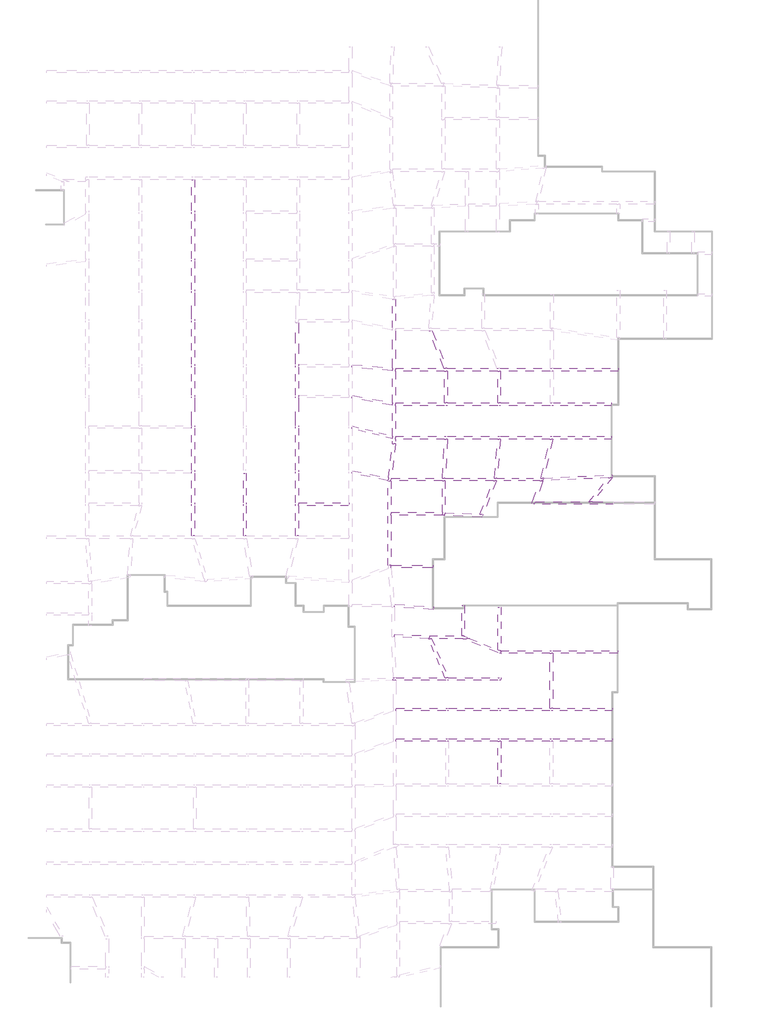
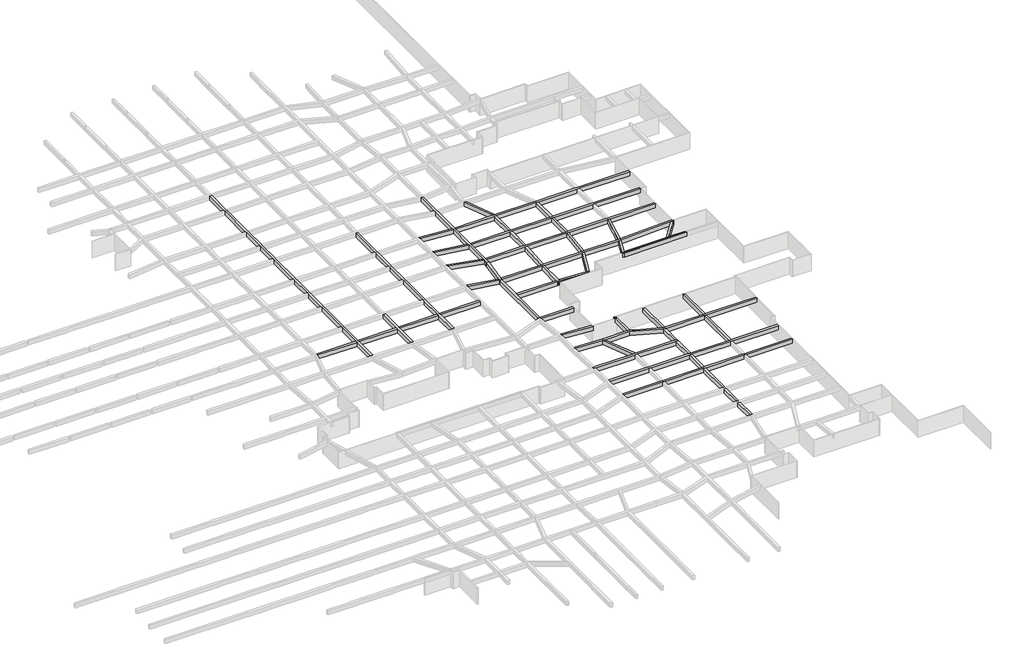
# One storey, part 24 of 45: 43 beams.
"""IFC4 building model written with IfcOpenShell, lengths in millimetres."""

from ifc_helpers import new_model, si_unit, frame, origin, place, context, project, spatial, polyline, outline, extrude, faceted_brep, element, save

model = new_model("IFC4")

# Units and contexts
model_context = context("Model", 3, world=origin())
ifc_project = project(units=[si_unit("LENGTHUNIT", "METRE", prefix="MILLI")], contexts=[model_context])

# Site, building, storey
site = spatial("IfcSite", under=ifc_project)
building = spatial("IfcBuilding", under=site)
storey = spatial("IfcBuildingStorey", under=building, Name="户型图", Elevation=0.0)

# Beams
placement = place(None, origin())
element("IfcBeam", 1, ObjectType="混凝土 - 矩形梁 : KL_beam", at=placement, inside=storey, context=model_context, shape_type="Brep", body=[
    faceted_brep([(1471.7652295, 23868.127427, 3300.0), (1071.7652295, 23868.127427, 3300.0), (1071.7652295, 19231.9876735, 3300.0), (1071.7652295, 18831.9876735, 3300.0), (1071.7652295, 12131.9876735, 3300.0), (1071.7652295, 11731.9876735, 3300.0), (1071.7652295, 7519.5822838, 3300.0), (1071.7652295, 7119.5822838, 3300.0), (1071.7652295, 3119.5822838, 3300.0), (1071.7652295, 2719.5822838, 3300.0), (1071.7652295, -3551.5199121, 3300.0), (1071.7652295, -3951.5199121, 3300.0), (1071.7652295, -8106.533538, 3300.0), (1071.7652295, -8506.533538, 3300.0), (1071.7652295, -12606.533538, 3300.0), (1071.7652295, -13006.533538, 3300.0), (1071.7652295, -19266.2432363, 3300.0), (1071.7652295, -19666.2432363, 3300.0), (1071.7652295, -24066.2432363, 3300.0), (1071.7652295, -24466.2432363, 3300.0), (1071.7652295, -28962.9587641, 3300.0), (1471.7652295, -28962.9587641, 3300.0), (1471.7652295, -24466.2432363, 3300.0), (1471.7652295, -24066.2432363, 3300.0), (1471.7652295, -19666.2432363, 3300.0), (1471.7652295, -19266.2432363, 3300.0), (1471.7652295, -13006.533538, 3300.0), (1471.7652295, -12606.533538, 3300.0), (1471.7652295, -8506.533538, 3300.0), (1471.7652295, -8106.533538, 3300.0), (1471.7652295, -3951.5199121, 3300.0), (1471.7652295, -3551.5199121, 3300.0), (1471.7652295, 2719.5822838, 3300.0), (1471.7652295, 3119.5822838, 3300.0), (1471.7652295, 7119.5822838, 3300.0), (1471.7652295, 7519.5822838, 3300.0), (1471.7652295, 11731.9876735, 3300.0), (1471.7652295, 12131.9876735, 3300.0), (1471.7652295, 18831.9876735, 3300.0), (1471.7652295, 19231.9876735, 3300.0), (1071.7652295, 23868.127427, 2500.0), (1071.7652295, 19231.9876735, 2500.0), (1071.7652295, 18831.9876735, 2500.0), (1071.7652295, 12131.9876735, 2500.0), (1071.7652295, 11731.9876735, 2500.0), (1071.7652295, 7519.5822838, 2500.0), (1071.7652295, 7119.5822838, 2500.0), (1071.7652295, 3119.5822838, 2500.0), (1071.7652295, 2719.5822838, 2500.0), (1071.7652295, -3551.5199121, 2500.0), (1071.7652295, -3951.5199121, 2500.0), (1071.7652295, -8106.533538, 2500.0), (1071.7652295, -8506.533538, 2500.0), (1071.7652295, -12606.533538, 2500.0), (1071.7652295, -13006.533538, 2500.0), (1071.7652295, -19266.2432363, 2500.0), (1071.7652295, -19666.2432363, 2500.0), (1071.7652295, -24066.2432363, 2500.0), (1071.7652295, -24466.2432363, 2500.0), (1071.7652295, -28962.9587641, 2500.0), (1471.7652295, 23868.127427, 2500.0), (1471.7652295, 19231.9876735, 2500.0), (1471.7652295, 18831.9876735, 2500.0), (1471.7652295, 12131.9876735, 2500.0), (1471.7652295, 11731.9876735, 2500.0), (1471.7652295, 7519.5822838, 2500.0), (1471.7652295, 7119.5822838, 2500.0), (1471.7652295, 3119.5822838, 2500.0), (1471.7652295, 2719.5822838, 2500.0), (1471.7652295, -3551.5199121, 2500.0), (1471.7652295, -3951.5199121, 2500.0), (1471.7652295, -8106.533538, 2500.0), (1471.7652295, -8506.533538, 2500.0), (1471.7652295, -12606.533538, 2500.0), (1471.7652295, -13006.533538, 2500.0), (1471.7652295, -19266.2432363, 2500.0), (1471.7652295, -19666.2432363, 2500.0), (1471.7652295, -24066.2432363, 2500.0), (1471.7652295, -24466.2432363, 2500.0), (1471.7652295, -28962.9587641, 2500.0)], [[[0, 1, 2, 3, 4, 5, 6, 7, 8, 9, 10, 11, 12, 13, 14, 15, 16, 17, 18, 19, 20, 21, 22, 23, 24, 25, 26, 27, 28, 29, 30, 31, 32, 33, 34, 35, 36, 37, 38, 39]], [[1, 40, 41, 42, 43, 44, 45, 46, 47, 48, 49, 50, 51, 52, 53, 54, 55, 56, 57, 58, 59, 20, 19, 18, 17, 16, 15, 14, 13, 12, 11, 10, 9, 8, 7, 6, 5, 4, 3, 2]], [[40, 60, 61, 62, 63, 64, 65, 66, 67, 68, 69, 70, 71, 72, 73, 74, 75, 76, 77, 78, 79, 59, 58, 57, 56, 55, 54, 53, 52, 51, 50, 49, 48, 47, 46, 45, 44, 43, 42, 41]], [[60, 0, 39, 38, 37, 36, 35, 34, 33, 32, 31, 30, 29, 28, 27, 26, 25, 24, 23, 22, 21, 79, 78, 77, 76, 75, 74, 73, 72, 71, 70, 69, 68, 67, 66, 65, 64, 63, 62, 61]], [[1, 0, 60, 40]], [[21, 20, 59, 79]]]),
])
element("IfcBeam", 2, ObjectType="混凝土 - 矩形梁 : KL_beam", at=placement, inside=storey, context=model_context, shape_type="Brep", body=[
    faceted_brep([(9169.3873949, -19666.2432363, 3300.0), (8769.3873949, -19666.2432363, 3300.0), (8769.3873949, -24066.2432363, 3300.0), (8769.3873949, -24466.2432363, 3300.0), (8769.3873949, -28962.9587641, 3300.0), (9169.3873949, -28962.9587641, 3300.0), (9169.3873949, -24466.2432363, 3300.0), (9169.3873949, -24066.2432363, 3300.0), (9169.3873949, -19666.2432363, 2500.0), (9169.3873949, -28962.9587641, 2500.0), (9169.3873949, -24466.2432363, 2500.0), (9169.3873949, -24066.2432363, 2500.0), (8769.3873949, -19666.2432363, 2500.0), (8769.3873949, -28962.9587641, 2500.0), (8769.3873949, -24466.2432363, 2500.0), (8769.3873949, -24066.2432363, 2500.0)], [[[0, 1, 2, 3, 4, 5, 6, 7]], [[8, 0, 7, 6, 5, 9, 10, 11]], [[12, 8, 11, 10, 9, 13, 14, 15]], [[1, 12, 15, 14, 13, 4, 3, 2]], [[1, 0, 8, 12]], [[5, 4, 13, 9]]]),
])
element("IfcBeam", 3, ObjectType="混凝土 - 矩形梁 : KL_beam", at=placement, inside=storey, context=model_context, shape_type="Brep", body=[
    faceted_brep([(16905.3597604, 2667.499527, 3300.0), (16505.3597604, 2674.481553, 3300.0), (16505.3597604, -3551.5199121, 3300.0), (16505.3597604, -3951.5199121, 3300.0), (16505.3597604, -8106.533538, 3300.0), (16505.3597604, -8506.533538, 3300.0), (16505.3597604, -12606.533538, 3300.0), (16505.3597604, -13006.533538, 3300.0), (16505.3597604, -19266.2432363, 3300.0), (16505.3597604, -19666.2432363, 3300.0), (16505.3597604, -24066.2432363, 3300.0), (16505.3597604, -24466.2432363, 3300.0), (16505.3597604, -28962.9587641, 3300.0), (16905.3597604, -28962.9587641, 3300.0), (16905.3597604, -24466.2432363, 3300.0), (16905.3597604, -24066.2432363, 3300.0), (16905.3597604, -19666.2432363, 3300.0), (16905.3597604, -19266.2432363, 3300.0), (16905.3597604, -13006.533538, 3300.0), (16905.3597604, -12606.533538, 3300.0), (16905.3597604, -8506.533538, 3300.0), (16905.3597604, -8106.533538, 3300.0), (16905.3597604, -3951.5199121, 3300.0), (16905.3597604, -3551.5199121, 3300.0), (16505.3597604, 2674.481553, 2500.0), (16505.3597604, -3551.5199121, 2500.0), (16505.3597604, -3951.5199121, 2500.0), (16505.3597604, -8106.533538, 2500.0), (16505.3597604, -8506.533538, 2500.0), (16505.3597604, -12606.533538, 2500.0), (16505.3597604, -13006.533538, 2500.0), (16505.3597604, -19266.2432363, 2500.0), (16505.3597604, -19666.2432363, 2500.0), (16505.3597604, -24066.2432363, 2500.0), (16505.3597604, -24466.2432363, 2500.0), (16505.3597604, -28962.9587641, 2500.0), (16905.3597604, 2667.499527, 2500.0), (16905.3597604, -3551.5199121, 2500.0), (16905.3597604, -3951.5199121, 2500.0), (16905.3597604, -8106.533538, 2500.0), (16905.3597604, -8506.533538, 2500.0), (16905.3597604, -12606.533538, 2500.0), (16905.3597604, -13006.533538, 2500.0), (16905.3597604, -19266.2432363, 2500.0), (16905.3597604, -19666.2432363, 2500.0), (16905.3597604, -24066.2432363, 2500.0), (16905.3597604, -24466.2432363, 2500.0), (16905.3597604, -28962.9587641, 2500.0)], [[[0, 1, 2, 3, 4, 5, 6, 7, 8, 9, 10, 11, 12, 13, 14, 15, 16, 17, 18, 19, 20, 21, 22, 23]], [[1, 24, 25, 26, 27, 28, 29, 30, 31, 32, 33, 34, 35, 12, 11, 10, 9, 8, 7, 6, 5, 4, 3, 2]], [[24, 36, 37, 38, 39, 40, 41, 42, 43, 44, 45, 46, 47, 35, 34, 33, 32, 31, 30, 29, 28, 27, 26, 25]], [[36, 0, 23, 22, 21, 20, 19, 18, 17, 16, 15, 14, 13, 47, 46, 45, 44, 43, 42, 41, 40, 39, 38, 37]], [[0, 36, 24, 1]], [[13, 12, 35, 47]]]),
])
element("IfcBeam", 4, ObjectType="混凝土 - 矩形梁 : KL_beam", at=placement, inside=storey, context=model_context, shape_type="SweptSolid", body=[
    extrude(outline(polyline([(-6328.2347705, -24466.2432363), (-6328.2347705, -24066.2432363), (1071.7652295, -24066.2432363), (1071.7652295, -24466.2432363), (-6328.2347705, -24466.2432363)])), frame((0.0, 0.0, 2500.0), z_axis=(0.0, 0.0, 1.0), x_axis=(1.0, 0.0, 0.0)), (0.0, 0.0, 1.0), 800.0),
    extrude(outline(polyline([(24442.7166646, -24066.2432363), (24442.7166646, -24466.2432363), (16905.3597604, -24466.2432363), (16905.3597604, -24066.2432363), (24442.7166646, -24066.2432363)])), frame((0.0, 0.0, 2500.0), z_axis=(0.0, 0.0, 1.0), x_axis=(1.0, 0.0, 0.0)), (0.0, 0.0, 1.0), 800.0),
    extrude(outline(polyline([(1471.7652295, -24466.2432363), (1471.7652295, -24066.2432363), (8769.3873949, -24066.2432363), (8769.3873949, -24466.2432363), (1471.7652295, -24466.2432363)])), frame((0.0, 0.0, 2500.0), z_axis=(0.0, 0.0, 1.0), x_axis=(1.0, 0.0, 0.0)), (0.0, 0.0, 1.0), 800.0),
    extrude(outline(polyline([(9169.3873949, -24466.2432363), (9169.3873949, -24066.2432363), (16505.3597604, -24066.2432363), (16505.3597604, -24466.2432363), (9169.3873949, -24466.2432363)])), frame((0.0, 0.0, 2500.0), z_axis=(0.0, 0.0, 1.0), x_axis=(1.0, 0.0, 0.0)), (0.0, 0.0, 1.0), 800.0),
])
element("IfcBeam", 5, ObjectType="混凝土 - 矩形梁 : KL_beam", at=placement, inside=storey, context=model_context, shape_type="Brep", body=[
    faceted_brep([(31293.5212654, -15309.9620605, 3300.0), (31293.5212654, -14614.9150331, 3300.0), (31293.5212654, -14214.9150331, 3300.0), (31293.5212654, -9661.6279316, 3300.0), (31293.5212654, -9261.6279316, 3300.0), (31293.5212654, -4524.63893, 3300.0), (31293.5212654, -4124.63893, 3300.0), (31293.5212654, 1446.1972666, 3300.0), (31293.5212654, 1846.1972666, 3300.0), (31293.5212654, 6125.9678564, 3300.0), (31056.9345953, 6101.1015953, 3300.0), (30993.5212654, 6111.1452801, 3300.0), (30893.5212654, 6126.9837241, 3300.0), (30893.5212654, 1908.2546983, 3300.0), (30893.5212654, 1500.7680203, 3300.0), (30893.5212654, -4097.664429, 3300.0), (30893.5212654, -4499.192364, 3300.0), (30893.5212654, -9205.644515, 3300.0), (30893.5212654, -9611.8151597, 3300.0), (30893.5212654, -14158.9267066, 3300.0), (30893.5212654, -14571.1721584, 3300.0), (30893.5212654, -15285.4970125, 3300.0), (30893.5212654, 6126.9837241, 2500.0), (30893.5212654, 1908.2546983, 2500.0), (30893.5212654, 1500.7680203, 2500.0), (30893.5212654, -4097.664429, 2500.0), (30893.5212654, -4499.192364, 2500.0), (30893.5212654, -9205.644515, 2500.0), (30893.5212654, -9611.8151597, 2500.0), (30893.5212654, -14158.9267066, 2500.0), (30893.5212654, -14571.1721584, 2500.0), (30893.5212654, -15285.4970125, 2500.0), (31293.5212654, 6125.9678564, 2500.0), (31293.5212654, 1846.1972666, 2500.0), (31293.5212654, 1446.1972666, 2500.0), (31293.5212654, -4124.63893, 2500.0), (31293.5212654, -4524.63893, 2500.0), (31293.5212654, -9261.6279316, 2500.0), (31293.5212654, -9661.6279316, 2500.0), (31293.5212654, -14214.9150331, 2500.0), (31293.5212654, -14614.9150331, 2500.0), (31293.5212654, -15309.9620605, 2500.0), (30993.5212654, 6111.1452801, 2500.0), (31056.9345953, 6101.1015953, 2500.0)], [[[0, 1, 2, 3, 4, 5, 6, 7, 8, 9, 10, 11, 12, 13, 14, 15, 16, 17, 18, 19, 20, 21]], [[21, 20, 19, 18, 17, 16, 15, 14, 13, 12, 22, 23, 24, 25, 26, 27, 28, 29, 30, 31]], [[32, 33, 34, 35, 36, 37, 38, 39, 40, 41, 31, 30, 29, 28, 27, 26, 25, 24, 23, 22, 42, 43]], [[9, 8, 7, 6, 5, 4, 3, 2, 1, 0, 41, 40, 39, 38, 37, 36, 35, 34, 33, 32]], [[10, 9, 32, 43]], [[22, 12, 11, 10, 43, 42]], [[0, 21, 31, 41]]]),
])
element("IfcBeam", 6, ObjectType="混凝土 - 矩形梁 : KL_beam", at=placement, inside=storey, context=model_context, shape_type="Brep", body=[
    faceted_brep([(30613.5574676, -20847.8227882, 3300.0), (30620.19498, -20793.7645877, 3300.0), (30669.3088044, -20393.7645877, 3300.0), (31293.5212654, -15309.9620605, 3300.0), (30893.5212654, -15285.4970125, 3300.0), (30270.8784709, -20356.5156317, 3300.0), (30222.0116965, -20754.503571, 3300.0), (30213.5574676, -20823.3577402, 3300.0), (30893.5212654, -15285.4970125, 2500.0), (30270.8784709, -20356.5156317, 2500.0), (30222.0116965, -20754.503571, 2500.0), (30213.5574676, -20823.3577402, 2500.0), (31293.5212654, -15309.9620605, 2500.0), (30669.3088044, -20393.7645877, 2500.0), (30620.19498, -20793.7645877, 2500.0), (30613.5574676, -20847.8227882, 2500.0)], [[[0, 1, 2, 3, 4, 5, 6, 7]], [[7, 6, 5, 4, 8, 9, 10, 11]], [[11, 10, 9, 8, 12, 13, 14, 15]], [[3, 2, 1, 0, 15, 14, 13, 12]], [[3, 12, 8, 4]], [[0, 7, 11, 15]]]),
])
element("IfcBeam", 7, ObjectType="混凝土 - 矩形梁 : KL_beam", at=placement, inside=storey, context=model_context, shape_type="Brep", body=[
    faceted_brep([(30613.5574676, -33326.8580756, 3300.0), (30613.5574676, -33322.5859731, 3300.0), (30613.5574676, -25893.7645877, 3300.0), (30613.5574676, -25493.7645877, 3300.0), (30613.5574676, -20847.8227882, 3300.0), (30213.5574676, -20823.3577402, 3300.0), (30213.5574676, -33322.5859731, 3300.0), (30213.5574676, -33344.3224528, 3300.0), (30213.5574676, -20823.3577402, 2500.0), (30213.5574676, -33322.5859731, 2500.0), (30213.5574676, -33344.3224528, 2500.0), (30613.5574676, -20847.8227882, 2500.0), (30613.5574676, -25493.7645877, 2500.0), (30613.5574676, -25893.7645877, 2500.0), (30613.5574676, -33322.5859731, 2500.0), (30613.5574676, -33326.8580756, 2500.0)], [[[0, 1, 2, 3, 4, 5, 6, 7]], [[7, 6, 5, 8, 9, 10]], [[10, 9, 8, 11, 12, 13, 14, 15]], [[4, 3, 2, 1, 0, 15, 14, 13, 12, 11]], [[4, 11, 8, 5]], [[0, 7, 10, 15]]]),
])
element("IfcBeam", 8, ObjectType="混凝土 - 矩形梁 : KL_beam", at=placement, inside=storey, context=model_context, shape_type="SweptSolid", body=[
    extrude(outline(polyline([(24842.7166646, -3969.8155562), (24842.7166646, -3568.2876212), (30893.5212654, -4097.664429), (30893.5212654, -4499.192364), (24842.7166646, -3969.8155562)])), frame((0.0, 0.0, 2500.0), z_axis=(0.0, 0.0, 1.0), x_axis=(1.0, 0.0, 0.0)), (0.0, 0.0, 1.0), 800.0),
])
element("IfcBeam", 9, ObjectType="混凝土 - 矩形梁 : KL_beam", at=placement, inside=storey, context=model_context, shape_type="Brep", body=[
    faceted_brep([(64358.9998045, -4124.63893, 3300.0), (64358.9998045, -4524.63893, 3300.0), (64358.9998045, -4524.63893, 2500.0), (64358.9998045, -4124.63893, 2500.0), (54693.5212654, -4124.63893, 3300.0), (54293.5212654, -4124.63893, 3300.0), (46792.4867011, -4124.63893, 3300.0), (46362.3003567, -4124.63893, 3300.0), (38929.4075897, -4124.63893, 3300.0), (38499.2212453, -4124.63893, 3300.0), (31293.5212654, -4124.63893, 3300.0), (31293.5212654, -4524.63893, 3300.0), (38593.5212654, -4524.63893, 3300.0), (38993.5212654, -4524.63893, 3300.0), (46493.5212654, -4524.63893, 3300.0), (46893.5212654, -4524.63893, 3300.0), (54293.5212654, -4524.63893, 3300.0), (54693.5212654, -4524.63893, 3300.0), (31293.5212654, -4524.63893, 2500.0), (38593.5212654, -4524.63893, 2500.0), (38993.5212654, -4524.63893, 2500.0), (46493.5212654, -4524.63893, 2500.0), (46893.5212654, -4524.63893, 2500.0), (54293.5212654, -4524.63893, 2500.0), (54693.5212654, -4524.63893, 2500.0), (31293.5212654, -4124.63893, 2500.0), (38499.2212453, -4124.63893, 2500.0), (38929.4075897, -4124.63893, 2500.0), (46362.3003567, -4124.63893, 2500.0), (46792.4867011, -4124.63893, 2500.0), (54293.5212654, -4124.63893, 2500.0), (54693.5212654, -4124.63893, 2500.0)], [[[0, 1, 2, 3]], [[1, 0, 4, 5, 6, 7, 8, 9, 10, 11, 12, 13, 14, 15, 16, 17]], [[2, 1, 17, 16, 15, 14, 13, 12, 11, 18, 19, 20, 21, 22, 23, 24]], [[3, 2, 24, 23, 22, 21, 20, 19, 18, 25, 26, 27, 28, 29, 30, 31]], [[0, 3, 31, 30, 29, 28, 27, 26, 25, 10, 9, 8, 7, 6, 5, 4]], [[11, 10, 25, 18]]]),
])
element("IfcBeam", 10, ObjectType="混凝土 - 矩形梁 : KL_beam", at=placement, inside=storey, context=model_context, shape_type="SweptSolid", body=[
    extrude(outline(polyline([(24842.7166646, -8544.8950536), (24842.7166646, -8138.7244089), (30893.5212654, -9205.644515), (30893.5212654, -9611.8151597), (24842.7166646, -8544.8950536)])), frame((0.0, 0.0, 2500.0), z_axis=(0.0, 0.0, 1.0), x_axis=(1.0, 0.0, 0.0)), (0.0, 0.0, 1.0), 800.0),
])
element("IfcBeam", 11, ObjectType="混凝土 - 矩形梁 : KL_beam", at=placement, inside=storey, context=model_context, shape_type="Brep", body=[
    faceted_brep([(63358.9998045, -9261.6279316, 3300.0), (63358.9998045, -9661.6279316, 3300.0), (63358.9998045, -9661.6279316, 2500.0), (63358.9998045, -9261.6279316, 2500.0), (54693.5212654, -9261.6279316, 3300.0), (54293.5212654, -9261.6279316, 3300.0), (46893.5212654, -9261.6279316, 3300.0), (46493.5212654, -9261.6279316, 3300.0), (38993.5212654, -9261.6279316, 3300.0), (38593.5212654, -9261.6279316, 3300.0), (31293.5212654, -9261.6279316, 3300.0), (31293.5212654, -9661.6279316, 3300.0), (38593.5212654, -9661.6279316, 3300.0), (38993.5212654, -9661.6279316, 3300.0), (46493.5212654, -9661.6279316, 3300.0), (46893.5212654, -9661.6279316, 3300.0), (54293.5212654, -9661.6279316, 3300.0), (54693.5212654, -9661.6279316, 3300.0), (31293.5212654, -9661.6279316, 2500.0), (38593.5212654, -9661.6279316, 2500.0), (38993.5212654, -9661.6279316, 2500.0), (46493.5212654, -9661.6279316, 2500.0), (46893.5212654, -9661.6279316, 2500.0), (54293.5212654, -9661.6279316, 2500.0), (54693.5212654, -9661.6279316, 2500.0), (31293.5212654, -9261.6279316, 2500.0), (38593.5212654, -9261.6279316, 2500.0), (38993.5212654, -9261.6279316, 2500.0), (46493.5212654, -9261.6279316, 2500.0), (46893.5212654, -9261.6279316, 2500.0), (54293.5212654, -9261.6279316, 2500.0), (54693.5212654, -9261.6279316, 2500.0)], [[[0, 1, 2, 3]], [[1, 0, 4, 5, 6, 7, 8, 9, 10, 11, 12, 13, 14, 15, 16, 17]], [[2, 1, 17, 16, 15, 14, 13, 12, 11, 18, 19, 20, 21, 22, 23, 24]], [[3, 2, 24, 23, 22, 21, 20, 19, 18, 25, 26, 27, 28, 29, 30, 31]], [[0, 3, 31, 30, 29, 28, 27, 26, 25, 10, 9, 8, 7, 6, 5, 4]], [[11, 10, 25, 18]]]),
])
element("IfcBeam", 12, ObjectType="混凝土 - 矩形梁 : KL_beam", at=placement, inside=storey, context=model_context, shape_type="SweptSolid", body=[
    extrude(outline(polyline([(24842.7166646, -13062.5371316), (24842.7166646, -12650.2916799), (30893.5212654, -14158.9267066), (30893.5212654, -14571.1721584), (24842.7166646, -13062.5371316)])), frame((0.0, 0.0, 2500.0), z_axis=(0.0, 0.0, 1.0), x_axis=(1.0, 0.0, 0.0)), (0.0, 0.0, 1.0), 800.0),
])
element("IfcBeam", 13, ObjectType="混凝土 - 矩形梁 : KL_beam", at=placement, inside=storey, context=model_context, shape_type="Brep", body=[
    faceted_brep([(63358.9998045, -14214.9150331, 3300.0), (63358.9998045, -14614.9150331, 3300.0), (63358.9998045, -14614.9150331, 2500.0), (63358.9998045, -14214.9150331, 2500.0), (54693.5212654, -14214.9150331, 3300.0), (54293.5212654, -14214.9150331, 3300.0), (46893.5212654, -14214.9150331, 3300.0), (46493.5212654, -14214.9150331, 3300.0), (38993.5212654, -14214.9150331, 3300.0), (38593.5212654, -14214.9150331, 3300.0), (31293.5212654, -14214.9150331, 3300.0), (31293.5212654, -14614.9150331, 3300.0), (38582.7580054, -14614.9150331, 3300.0), (38983.3069438, -14614.9150331, 3300.0), (46475.2595652, -14614.9150331, 3300.0), (46876.7875002, -14614.9150331, 3300.0), (54241.1117877, -14614.9150331, 3300.0), (54651.9818639, -14614.9150331, 3300.0), (31293.5212654, -14614.9150331, 2500.0), (38582.7580054, -14614.9150331, 2500.0), (38983.3069438, -14614.9150331, 2500.0), (46475.2595652, -14614.9150331, 2500.0), (46876.7875002, -14614.9150331, 2500.0), (54241.1117877, -14614.9150331, 2500.0), (54651.9818639, -14614.9150331, 2500.0), (31293.5212654, -14214.9150331, 2500.0), (38593.5212654, -14214.9150331, 2500.0), (38993.5212654, -14214.9150331, 2500.0), (46493.5212654, -14214.9150331, 2500.0), (46893.5212654, -14214.9150331, 2500.0), (54293.5212654, -14214.9150331, 2500.0), (54693.5212654, -14214.9150331, 2500.0)], [[[0, 1, 2, 3]], [[1, 0, 4, 5, 6, 7, 8, 9, 10, 11, 12, 13, 14, 15, 16, 17]], [[2, 1, 17, 16, 15, 14, 13, 12, 11, 18, 19, 20, 21, 22, 23, 24]], [[3, 2, 24, 23, 22, 21, 20, 19, 18, 25, 26, 27, 28, 29, 30, 31]], [[0, 3, 31, 30, 29, 28, 27, 26, 25, 10, 9, 8, 7, 6, 5, 4]], [[11, 10, 25, 18]]]),
])
element("IfcBeam", 14, ObjectType="混凝土 - 矩形梁 : KL_beam", at=placement, inside=storey, context=model_context, shape_type="SweptSolid", body=[
    extrude(outline(polyline([(38593.5212654, -4524.63893), (38993.5212654, -4524.63893), (38993.5212654, -9261.6279316), (38593.5212654, -9261.6279316), (38593.5212654, -4524.63893)])), frame((0.0, 0.0, 2500.0), z_axis=(0.0, 0.0, 1.0), x_axis=(1.0, 0.0, 0.0)), (0.0, 0.0, 1.0), 800.0),
    extrude(outline(polyline([(38993.5212654, -14214.9150331), (38593.5212654, -14214.9150331), (38593.5212654, -9661.6279316), (38993.5212654, -9661.6279316), (38993.5212654, -14214.9150331)])), frame((0.0, 0.0, 2500.0), z_axis=(0.0, 0.0, 1.0), x_axis=(1.0, 0.0, 0.0)), (0.0, 0.0, 1.0), 800.0),
])
element("IfcBeam", 15, ObjectType="混凝土 - 矩形梁 : KL_beam", at=placement, inside=storey, context=model_context, shape_type="SweptSolid", body=[
    extrude(outline(polyline([(46493.5212654, -4524.63893), (46893.5212654, -4524.63893), (46893.5212654, -9261.6279316), (46493.5212654, -9261.6279316), (46493.5212654, -4524.63893)])), frame((0.0, 0.0, 2500.0), z_axis=(0.0, 0.0, 1.0), x_axis=(1.0, 0.0, 0.0)), (0.0, 0.0, 1.0), 800.0),
    extrude(outline(polyline([(46893.5212654, -14214.9150331), (46493.5212654, -14214.9150331), (46493.5212654, -9661.6279316), (46893.5212654, -9661.6279316), (46893.5212654, -14214.9150331)])), frame((0.0, 0.0, 2500.0), z_axis=(0.0, 0.0, 1.0), x_axis=(1.0, 0.0, 0.0)), (0.0, 0.0, 1.0), 800.0),
])
element("IfcBeam", 16, ObjectType="混凝土 - 矩形梁 : KL_beam", at=placement, inside=storey, context=model_context, shape_type="SweptSolid", body=[
    extrude(outline(polyline([(36294.5011943, 1446.1972666), (36724.6875387, 1446.1972666), (38929.4075897, -4124.63893), (38499.2212453, -4124.63893), (36294.5011943, 1446.1972666)])), frame((0.0, 0.0, 2500.0), z_axis=(0.0, 0.0, 1.0), x_axis=(1.0, 0.0, 0.0)), (0.0, 0.0, 1.0), 800.0),
])
element("IfcBeam", 17, ObjectType="混凝土 - 矩形梁 : KL_beam", at=placement, inside=storey, context=model_context, shape_type="Brep", body=[
    faceted_brep([(63459.3057658, -59021.1336343, 3300.0), (63459.3057658, -59421.1336343, 3300.0), (63459.3057658, -59421.1336343, 2500.0), (63459.3057658, -59021.1336343, 2500.0), (54624.1889168, -59021.1336343, 3300.0), (54224.1889168, -59021.1336343, 3300.0), (46924.1889168, -59021.1336343, 3300.0), (46524.1889168, -59021.1336343, 3300.0), (39180.1331881, -59021.1336343, 3300.0), (38780.1331881, -59021.1336343, 3300.0), (31380.1331881, -59021.1336343, 3300.0), (31380.1331881, -59421.1336343, 3300.0), (38780.1331881, -59421.1336343, 3300.0), (39180.1331881, -59421.1336343, 3300.0), (46524.1889168, -59421.1336343, 3300.0), (46924.1889168, -59421.1336343, 3300.0), (54224.1889168, -59421.1336343, 3300.0), (54624.1889168, -59421.1336343, 3300.0), (31380.1331881, -59421.1336343, 2500.0), (38780.1331881, -59421.1336343, 2500.0), (39180.1331881, -59421.1336343, 2500.0), (46524.1889168, -59421.1336343, 2500.0), (46924.1889168, -59421.1336343, 2500.0), (54224.1889168, -59421.1336343, 2500.0), (54624.1889168, -59421.1336343, 2500.0), (31380.1331881, -59021.1336343, 2500.0), (38780.1331881, -59021.1336343, 2500.0), (39180.1331881, -59021.1336343, 2500.0), (46524.1889168, -59021.1336343, 2500.0), (46924.1889168, -59021.1336343, 2500.0), (54224.1889168, -59021.1336343, 2500.0), (54624.1889168, -59021.1336343, 2500.0)], [[[0, 1, 2, 3]], [[1, 0, 4, 5, 6, 7, 8, 9, 10, 11, 12, 13, 14, 15, 16, 17]], [[2, 1, 17, 16, 15, 14, 13, 12, 11, 18, 19, 20, 21, 22, 23, 24]], [[3, 2, 24, 23, 22, 21, 20, 19, 18, 25, 26, 27, 28, 29, 30, 31]], [[0, 3, 31, 30, 29, 28, 27, 26, 25, 10, 9, 8, 7, 6, 5, 4]], [[10, 25, 18, 11]]]),
])
element("IfcBeam", 18, ObjectType="混凝土 - 矩形梁 : KL_beam", at=placement, inside=storey, context=model_context, shape_type="Brep", body=[
    faceted_brep([(63459.3057658, -54489.5663744, 3300.0), (63459.3057658, -54889.5663744, 3300.0), (63459.3057658, -54889.5663744, 2500.0), (63459.3057658, -54489.5663744, 2500.0), (54624.1889168, -54489.5663744, 3300.0), (54224.1889168, -54489.5663744, 3300.0), (46924.1889168, -54489.5663744, 3300.0), (46524.1889168, -54489.5663744, 3300.0), (39180.1331881, -54489.5663744, 3300.0), (38780.1331881, -54489.5663744, 3300.0), (31380.1331881, -54489.5663744, 3300.0), (31380.1331881, -54889.5663744, 3300.0), (38780.1331881, -54889.5663744, 3300.0), (39180.1331881, -54889.5663744, 3300.0), (46524.1889168, -54889.5663744, 3300.0), (46924.1889168, -54889.5663744, 3300.0), (54224.1889168, -54889.5663744, 3300.0), (54624.1889168, -54889.5663744, 3300.0), (31380.1331881, -54889.5663744, 2500.0), (38780.1331881, -54889.5663744, 2500.0), (39180.1331881, -54889.5663744, 2500.0), (46524.1889168, -54889.5663744, 2500.0), (46924.1889168, -54889.5663744, 2500.0), (54224.1889168, -54889.5663744, 2500.0), (54624.1889168, -54889.5663744, 2500.0), (31380.1331881, -54489.5663744, 2500.0), (38780.1331881, -54489.5663744, 2500.0), (39180.1331881, -54489.5663744, 2500.0), (46524.1889168, -54489.5663744, 2500.0), (46924.1889168, -54489.5663744, 2500.0), (54224.1889168, -54489.5663744, 2500.0), (54624.1889168, -54489.5663744, 2500.0)], [[[0, 1, 2, 3]], [[1, 0, 4, 5, 6, 7, 8, 9, 10, 11, 12, 13, 14, 15, 16, 17]], [[2, 1, 17, 16, 15, 14, 13, 12, 11, 18, 19, 20, 21, 22, 23, 24]], [[3, 2, 24, 23, 22, 21, 20, 19, 18, 25, 26, 27, 28, 29, 30, 31]], [[0, 3, 31, 30, 29, 28, 27, 26, 25, 10, 9, 8, 7, 6, 5, 4]], [[10, 25, 18, 11]]]),
])
element("IfcBeam", 19, ObjectType="混凝土 - 矩形梁 : KL_beam", at=placement, inside=storey, context=model_context, shape_type="Brep", body=[
    faceted_brep([(46953.9230726, -49989.5663744, 3300.0), (46953.9230726, -50389.5663744, 3300.0), (46953.9230726, -50389.5663744, 2500.0), (46953.9230726, -49989.5663744, 2500.0), (30953.9230726, -49989.5663744, 3300.0), (30953.9230726, -49989.5663744, 2500.0), (30953.9230726, -49997.3436027, 2500.0), (30953.9230726, -50389.5663744, 2500.0), (30953.9230726, -50389.5663744, 3300.0), (30953.9230726, -49997.3436027, 3300.0), (46924.1889168, -49989.5663744, 3300.0), (46524.1889168, -49989.5663744, 3300.0), (39112.43149, -49989.5663744, 3300.0), (38677.7861479, -49989.5663744, 3300.0), (31373.2625209, -49989.5663744, 3300.0), (30973.0187032, -49989.5663744, 3300.0), (30980.1331881, -50389.5663744, 3300.0), (31380.1331881, -50389.5663744, 3300.0), (38780.1331881, -50389.5663744, 3300.0), (39180.1331881, -50389.5663744, 3300.0), (46524.1889168, -50389.5663744, 3300.0), (46924.1889168, -50389.5663744, 3300.0), (30980.1331881, -50389.5663744, 2500.0), (31380.1331881, -50389.5663744, 2500.0), (38780.1331881, -50389.5663744, 2500.0), (39180.1331881, -50389.5663744, 2500.0), (46524.1889168, -50389.5663744, 2500.0), (46924.1889168, -50389.5663744, 2500.0), (30973.0187032, -49989.5663744, 2500.0), (31373.2625209, -49989.5663744, 2500.0), (38677.7861479, -49989.5663744, 2500.0), (39112.43149, -49989.5663744, 2500.0), (46524.1889168, -49989.5663744, 2500.0), (46924.1889168, -49989.5663744, 2500.0)], [[[0, 1, 2, 3]], [[4, 5, 6, 7, 8, 9]], [[1, 0, 10, 11, 12, 13, 14, 15, 4, 9, 8, 16, 17, 18, 19, 20, 21]], [[2, 1, 21, 20, 19, 18, 17, 16, 8, 7, 22, 23, 24, 25, 26, 27]], [[3, 2, 27, 26, 25, 24, 23, 22, 7, 6, 5, 28, 29, 30, 31, 32, 33]], [[0, 3, 33, 32, 31, 30, 29, 28, 5, 4, 15, 14, 13, 12, 11, 10]]]),
])
element("IfcBeam", 20, ObjectType="混凝土 - 矩形梁 : KL_beam", at=placement, inside=storey, context=model_context, shape_type="Brep", body=[
    faceted_brep([(36341.285376, -44194.6115561, 3300.0), (36351.7597446, -43794.6115561, 3300.0), (31153.9230726, -43522.204479, 3300.0), (31153.9230726, -43922.7534174, 3300.0), (31161.4184615, -43923.1462341, 3300.0), (36211.3288675, -44187.8008241, 3300.0), (36341.285376, -44194.6115561, 2500.0), (31153.9230726, -43922.7534174, 2500.0), (31161.4184615, -43923.1462341, 2500.0), (36211.3288675, -44187.8008241, 2500.0), (36351.7597446, -43794.6115561, 2500.0), (31153.9230726, -43522.204479, 2500.0)], [[[0, 1, 2, 3, 4, 5]], [[6, 0, 5, 4, 3, 7, 8, 9]], [[10, 6, 9, 8, 7, 11]], [[1, 10, 11, 2]], [[3, 2, 11, 7]], [[1, 0, 6, 10]]]),
])
element("IfcBeam", 21, ObjectType="混凝土 - 矩形梁 : KL_beam", at=placement, inside=storey, context=model_context, shape_type="Brep", body=[
    faceted_brep([(36351.7597446, -43794.6115561, 3300.0), (36341.285376, -44194.6115561, 3300.0), (36648.8696006, -44194.6115561, 3300.0), (41307.6464985, -44194.6115561, 3300.0), (42375.4333635, -44194.6115561, 3300.0), (41546.5225603, -43859.7098527, 3300.0), (41385.3986221, -43794.6115561, 3300.0), (41146.5225603, -43794.6115561, 3300.0), (36341.285376, -44194.6115561, 2500.0), (36648.8696006, -44194.6115561, 2500.0), (41307.6464985, -44194.6115561, 2500.0), (42375.4333635, -44194.6115561, 2500.0), (36351.7597446, -43794.6115561, 2500.0), (41146.5225603, -43794.6115561, 2500.0), (41385.3986221, -43794.6115561, 2500.0), (41546.5225603, -43859.7098527, 2500.0)], [[[0, 1, 2, 3, 4, 5, 6, 7]], [[1, 8, 9, 10, 11, 4, 3, 2]], [[8, 12, 13, 14, 15, 11, 10, 9]], [[12, 0, 7, 6, 14, 13]], [[0, 12, 8, 1]], [[6, 5, 4, 11, 15, 14]]]),
])
element("IfcBeam", 22, ObjectType="混凝土 - 矩形梁 : KL_beam", at=placement, inside=storey, context=model_context, shape_type="Brep", body=[
    faceted_brep([(46924.1889168, -46463.8419916, 3300.0), (46924.1889168, -46367.3297979, 3300.0), (46924.1889168, -46032.4280945, 3300.0), (46763.0649786, -45967.3297979, 3300.0), (46524.3336302, -45870.8760722, 3300.0), (42375.4333635, -44194.6115561, 3300.0), (41307.6464985, -44194.6115561, 3300.0), (46524.1889168, -46302.2315013, 3300.0), (46924.1889168, -46463.8419916, 2500.0), (41307.6464985, -44194.6115561, 2500.0), (46524.1889168, -46302.2315013, 2500.0), (46924.1889168, -46032.4280945, 2500.0), (46924.1889168, -46367.3297979, 2500.0), (42375.4333635, -44194.6115561, 2500.0), (46524.3336302, -45870.8760722, 2500.0), (46763.0649786, -45967.3297979, 2500.0)], [[[0, 1, 2, 3, 4, 5, 6, 7]], [[8, 0, 7, 6, 9, 10]], [[11, 12, 8, 10, 9, 13, 14, 15]], [[2, 11, 15, 14, 13, 5, 4, 3]], [[6, 5, 13, 9]], [[2, 1, 0, 8, 12, 11]]]),
])
element("IfcBeam", 23, ObjectType="混凝土 - 矩形梁 : KL_beam", at=placement, inside=storey, context=model_context, shape_type="SweptSolid", body=[
    extrude(outline(polyline([(36211.3288675, -44187.8008241), (36341.285376, -44194.6115561), (36648.8696006, -44194.6115561), (39112.43149, -49989.5663744), (38677.7861479, -49989.5663744), (36211.3288675, -44187.8008241)])), frame((0.0, 0.0, 2500.0), z_axis=(0.0, 0.0, 1.0), x_axis=(1.0, 0.0, 0.0)), (0.0, 0.0, 1.0), 800.0),
])
element("IfcBeam", 24, ObjectType="混凝土 - 矩形梁 : KL_beam", at=placement, inside=storey, context=model_context, shape_type="SweptSolid", body=[
    extrude(outline(polyline([(46524.1889168, -46302.2315013), (46924.1889168, -46463.8419916), (46924.1889168, -49989.5663744), (46524.1889168, -49989.5663744), (46524.1889168, -46302.2315013)])), frame((0.0, 0.0, 2500.0), z_axis=(0.0, 0.0, 1.0), x_axis=(1.0, 0.0, 0.0)), (0.0, 0.0, 1.0), 800.0),
    extrude(outline(polyline([(46924.1889168, -74711.0797773), (46524.1889168, -74711.0797773), (46524.1889168, -70588.5460678), (46924.1889168, -70588.5460678), (46924.1889168, -74711.0797773)])), frame((0.0, 0.0, 2500.0), z_axis=(0.0, 0.0, 1.0), x_axis=(1.0, 0.0, 0.0)), (0.0, 0.0, 1.0), 800.0),
    extrude(outline(polyline([(46924.1889168, -70188.5460678), (46524.1889168, -70188.5460678), (46524.1889168, -66111.9700913), (46924.1889168, -66111.9700913), (46924.1889168, -70188.5460678)])), frame((0.0, 0.0, 2500.0), z_axis=(0.0, 0.0, 1.0), x_axis=(1.0, 0.0, 0.0)), (0.0, 0.0, 1.0), 800.0),
    extrude(outline(polyline([(46524.1889168, -65711.9700913), (46524.1889168, -59421.1336343), (46924.1889168, -59421.1336343), (46924.1889168, -65711.9700913), (46524.1889168, -65711.9700913)])), frame((0.0, 0.0, 2500.0), z_axis=(0.0, 0.0, 1.0), x_axis=(1.0, 0.0, 0.0)), (0.0, 0.0, 1.0), 800.0),
    extrude(outline(polyline([(46524.1889168, -59021.1336343), (46524.1889168, -54889.5663744), (46924.1889168, -54889.5663744), (46924.1889168, -59021.1336343), (46524.1889168, -59021.1336343)])), frame((0.0, 0.0, 2500.0), z_axis=(0.0, 0.0, 1.0), x_axis=(1.0, 0.0, 0.0)), (0.0, 0.0, 1.0), 800.0),
    extrude(outline(polyline([(46924.1889168, -54489.5663744), (46524.1889168, -54489.5663744), (46524.1889168, -50389.5663744), (46924.1889168, -50389.5663744), (46924.1889168, -54489.5663744)])), frame((0.0, 0.0, 2500.0), z_axis=(0.0, 0.0, 1.0), x_axis=(1.0, 0.0, 0.0)), (0.0, 0.0, 1.0), 800.0),
])
element("IfcBeam", 25, ObjectType="混凝土 - 矩形梁 : KL_beam", at=placement, inside=storey, context=model_context, shape_type="SweptSolid", body=[
    extrude(outline(polyline([(36932.8592041, -39497.8564742), (36904.9566146, -39896.8820943), (31166.6689283, -39495.6219304), (31194.5715178, -39096.5963103), (36932.8592041, -39497.8564742)])), frame((0.0, 0.0, 2500.0), z_axis=(0.0, 0.0, 1.0), x_axis=(1.0, 0.0, 0.0)), (0.0, 0.0, 1.0), 800.0),
])
element("IfcBeam", 26, ObjectType="混凝土 - 矩形梁 : KL_beam", at=placement, inside=storey, context=model_context, shape_type="Brep", body=[
    faceted_brep([(36829.9174723, -33322.5859731, 3300.0), (36829.9174723, -33722.5859731, 3300.0), (36829.9174723, -33722.5859731, 2500.0), (36829.9174723, -33322.5859731, 2500.0), (30613.5574676, -33322.5859731, 3300.0), (30613.5574676, -33326.8580756, 3300.0), (30623.4014797, -33439.3756487, 3300.0), (30642.2917245, -33655.2921345, 3300.0), (30648.1791725, -33722.5859731, 3300.0), (30648.1791725, -33722.5859731, 2500.0), (30642.2917245, -33655.2921345, 2500.0), (30623.4014797, -33439.3756487, 2500.0), (30613.5574676, -33326.8580756, 2500.0), (30613.5574676, -33322.5859731, 2500.0)], [[[0, 1, 2, 3]], [[1, 0, 4, 5, 6, 7, 8]], [[2, 1, 8, 9]], [[3, 2, 9, 10, 11, 12, 13]], [[0, 3, 13, 4]], [[9, 8, 7, 6, 5, 12, 11, 10]], [[5, 4, 13, 12]]]),
    faceted_brep([(30211.655772, -33322.5859731, 3300.0), (30211.655772, -33322.5859731, 2500.0), (30213.5574676, -33344.3224528, 2500.0), (30213.5574676, -33344.3224528, 3300.0), (30213.5574676, -33322.5859731, 3300.0), (30213.5574676, -33322.5859731, 2500.0)], [[[0, 1, 2, 3]], [[4, 3, 2, 5]], [[0, 3, 4]], [[2, 1, 5]], [[1, 0, 4, 5]]]),
])
element("IfcBeam", 27, ObjectType="混凝土 - 矩形梁 : KL_beam", at=placement, inside=storey, context=model_context, shape_type="SweptSolid", body=[
    extrude(outline(polyline([(24842.7166646, -19708.8745398), (24842.7166646, -19301.3878618), (30270.8784709, -20356.5156317), (30222.0116965, -20754.503571), (24842.7166646, -19708.8745398)])), frame((0.0, 0.0, 2500.0), z_axis=(0.0, 0.0, 1.0), x_axis=(1.0, 0.0, 0.0)), (0.0, 0.0, 1.0), 800.0),
])
element("IfcBeam", 28, ObjectType="混凝土 - 矩形梁 : KL_beam", at=placement, inside=storey, context=model_context, shape_type="Brep", body=[
    faceted_brep([(53201.7429278, -20793.7645877, 3300.0), (53203.3920711, -20786.7382912, 3300.0), (53295.6270027, -20393.7645877, 3300.0), (52884.7569265, -20393.7645877, 3300.0), (46371.2036759, -20393.7645877, 3300.0), (45969.6757409, -20393.7645877, 3300.0), (38680.4502718, -20393.7645877, 3300.0), (38279.9013334, -20393.7645877, 3300.0), (30669.3088044, -20393.7645877, 3300.0), (30664.4881577, -20433.0256043, 3300.0), (30620.19498, -20793.7645877, 3300.0), (38269.6942467, -20793.7645877, 3300.0), (38669.6942467, -20793.7645877, 3300.0), (45855.7999521, -20793.7645877, 3300.0), (46287.6054183, -20793.7645877, 3300.0), (52757.6353657, -20793.7645877, 3300.0), (53183.3064747, -20793.7645877, 3300.0), (30620.19498, -20793.7645877, 2500.0), (38269.6942467, -20793.7645877, 2500.0), (38669.6942467, -20793.7645877, 2500.0), (45855.7999521, -20793.7645877, 2500.0), (46287.6054183, -20793.7645877, 2500.0), (52757.6353657, -20793.7645877, 2500.0), (53183.3064747, -20793.7645877, 2500.0), (53201.7429278, -20793.7645877, 2500.0), (53295.6270027, -20393.7645877, 2500.0), (53203.3920711, -20786.7382912, 2500.0), (30664.4881577, -20433.0256043, 2500.0), (30669.3088044, -20393.7645877, 2500.0), (38279.9013334, -20393.7645877, 2500.0), (38680.4502718, -20393.7645877, 2500.0), (45969.6757409, -20393.7645877, 2500.0), (46371.2036759, -20393.7645877, 2500.0), (52884.7569265, -20393.7645877, 2500.0)], [[[0, 1, 2, 3, 4, 5, 6, 7, 8, 9, 10, 11, 12, 13, 14, 15, 16]], [[10, 17, 18, 19, 20, 21, 22, 23, 24, 0, 16, 15, 14, 13, 12, 11]], [[25, 26, 24, 23, 22, 21, 20, 19, 18, 17, 27, 28, 29, 30, 31, 32, 33]], [[28, 8, 7, 6, 5, 4, 3, 2, 25, 33, 32, 31, 30, 29]], [[17, 10, 9, 8, 28, 27]], [[2, 1, 0, 24, 26, 25]]]),
])
element("IfcBeam", 29, ObjectType="混凝土 - 矩形梁 : KL_beam", at=placement, inside=storey, context=model_context, shape_type="Brep", body=[
    faceted_brep([(52884.7569265, -20393.7645877, 3300.0), (53295.6270027, -20393.7645877, 3300.0), (53298.3783091, -20382.0424445, 3300.0), (54651.9818639, -14614.9150331, 3300.0), (54241.1117877, -14614.9150331, 3300.0), (53295.6270027, -20393.7645877, 2500.0), (53298.3783091, -20382.0424445, 2500.0), (54651.9818639, -14614.9150331, 2500.0), (52884.7569265, -20393.7645877, 2500.0), (54241.1117877, -14614.9150331, 2500.0)], [[[0, 1, 2, 3, 4]], [[1, 5, 6, 7, 3, 2]], [[5, 8, 9, 7, 6]], [[8, 0, 4, 9]], [[1, 0, 8, 5]], [[4, 3, 7, 9]]]),
])
element("IfcBeam", 30, ObjectType="混凝土 - 矩形梁 : KL_beam", at=placement, inside=storey, context=model_context, shape_type="SweptSolid", body=[
    extrude(outline(polyline([(46475.2595652, -14614.9150331), (46876.7875002, -14614.9150331), (46371.2036759, -20393.7645877), (45969.6757409, -20393.7645877), (46475.2595652, -14614.9150331)])), frame((0.0, 0.0, 2500.0), z_axis=(0.0, 0.0, 1.0), x_axis=(1.0, 0.0, 0.0)), (0.0, 0.0, 1.0), 800.0),
])
element("IfcBeam", 31, ObjectType="混凝土 - 矩形梁 : KL_beam", at=placement, inside=storey, context=model_context, shape_type="SweptSolid", body=[
    extrude(outline(polyline([(38582.7580054, -14614.9150331), (38983.3069438, -14614.9150331), (38680.4502718, -20393.7645877), (38279.9013334, -20393.7645877), (38582.7580054, -14614.9150331)])), frame((0.0, 0.0, 2500.0), z_axis=(0.0, 0.0, 1.0), x_axis=(1.0, 0.0, 0.0)), (0.0, 0.0, 1.0), 800.0),
])
element("IfcBeam", 32, ObjectType="混凝土 - 矩形梁 : KL_beam", at=placement, inside=storey, context=model_context, shape_type="Brep", body=[
    faceted_brep([(38269.6942467, -25893.7645877, 3300.0), (38464.4570624, -25893.7645877, 3300.0), (38669.6942467, -25893.7645877, 3300.0), (38669.6942467, -25503.9716743, 3300.0), (38669.6942467, -20793.7645877, 3300.0), (38269.6942467, -20793.7645877, 3300.0), (38269.6942467, -25493.7645877, 3300.0), (38269.6942467, -25893.7645877, 2500.0), (38269.6942467, -20793.7645877, 2500.0), (38269.6942467, -25493.7645877, 2500.0), (38669.6942467, -25893.7645877, 2500.0), (38464.4570624, -25893.7645877, 2500.0), (38669.6942467, -20793.7645877, 2500.0), (38669.6942467, -25503.9716743, 2500.0)], [[[0, 1, 2, 3, 4, 5, 6]], [[7, 0, 6, 5, 8, 9]], [[10, 11, 7, 9, 8, 12, 13]], [[2, 10, 13, 12, 4, 3]], [[5, 4, 12, 8]], [[2, 1, 0, 7, 11, 10]]]),
])
element("IfcBeam", 33, ObjectType="混凝土 - 矩形梁 : KL_beam", at=placement, inside=storey, context=model_context, shape_type="SweptSolid", body=[
    extrude(outline(polyline([(38269.6942467, -25493.7645877), (38269.6942467, -25893.7645877), (30613.5574676, -25893.7645877), (30613.5574676, -25493.7645877), (38269.6942467, -25493.7645877)])), frame((0.0, 0.0, 2500.0), z_axis=(0.0, 0.0, 1.0), x_axis=(1.0, 0.0, 0.0)), (0.0, 0.0, 1.0), 800.0),
])
element("IfcBeam", 34, ObjectType="混凝土 - 矩形梁 : KL_beam", at=placement, inside=storey, context=model_context, shape_type="Brep", body=[
    faceted_brep([(38669.6942467, -25503.9716743, 3300.0), (38669.6942467, -25893.7645877, 3300.0), (38464.4570624, -25893.7645877, 3300.0), (44093.815628, -26188.7867689, 3300.0), (44253.2931517, -25796.5956934, 3300.0), (43830.4977477, -25774.4379251, 3300.0), (38464.4570624, -25893.7645877, 2500.0), (44093.815628, -26188.7867689, 2500.0), (38669.6942467, -25893.7645877, 2500.0), (38669.6942467, -25503.9716743, 2500.0), (43830.4977477, -25774.4379251, 2500.0), (44253.2931517, -25796.5956934, 2500.0)], [[[0, 1, 2, 3, 4, 5]], [[2, 6, 7, 3]], [[8, 9, 10, 11, 7, 6]], [[9, 0, 5, 4, 11, 10]], [[8, 1, 0, 9]], [[1, 8, 6, 2]], [[4, 3, 7, 11]]]),
])
element("IfcBeam", 35, ObjectType="混凝土 - 矩形梁 : KL_beam", at=placement, inside=storey, context=model_context, shape_type="SweptSolid", body=[
    extrude(outline(polyline([(44253.2931517, -25796.5956934), (43830.4977477, -25774.4379251), (45855.7999521, -20793.7645877), (46287.6054183, -20793.7645877), (44253.2931517, -25796.5956934)])), frame((0.0, 0.0, 2500.0), z_axis=(0.0, 0.0, 1.0), x_axis=(1.0, 0.0, 0.0)), (0.0, 0.0, 1.0), 800.0),
])
element("IfcBeam", 36, ObjectType="混凝土 - 矩形梁 : KL_beam", at=placement, inside=storey, context=model_context, shape_type="Brep", body=[
    faceted_brep([(51541.9125467, -24133.9355811, 3300.0), (51917.789595, -24270.7436384, 3300.0), (52063.3776887, -23870.7436384, 3300.0), (53183.3064747, -20793.7645877, 3300.0), (53047.7623821, -20793.7645877, 3300.0), (52790.8728515, -20793.7645877, 3300.0), (52757.6353657, -20793.7645877, 3300.0), (52757.6353657, -20793.7645877, 2500.0), (51541.9125467, -24133.9355811, 2500.0), (51917.789595, -24270.7436384, 2500.0), (52790.8728515, -20793.7645877, 2500.0), (53047.7623821, -20793.7645877, 2500.0), (53183.3064747, -20793.7645877, 2500.0), (52063.3776887, -23870.7436384, 2500.0)], [[[0, 1, 2, 3, 4, 5, 6]], [[6, 7, 8, 0]], [[9, 8, 7, 10, 11, 12, 13]], [[12, 3, 2, 1, 9, 13]], [[7, 6, 5, 4, 3, 12, 11, 10]], [[1, 0, 8, 9]]]),
])
element("IfcBeam", 37, ObjectType="混凝土 - 矩形梁 : KL_beam", at=placement, inside=storey, context=model_context, shape_type="Brep", body=[
    faceted_brep([(53298.3783091, -20382.0424445, 3300.0), (53295.6270027, -20393.7645877, 3300.0), (53203.3920711, -20786.7382912, 3300.0), (62914.4439378, -20348.3082581, 3300.0), (63456.1178431, -20323.8530177, 3300.0), (63438.0772068, -19924.2600555, 3300.0), (53203.3920711, -20786.7382912, 2500.0), (62914.4439378, -20348.3082581, 2500.0), (63456.1178431, -20323.8530177, 2500.0), (53295.6270027, -20393.7645877, 2500.0), (53298.3783091, -20382.0424445, 2500.0), (63438.0772068, -19924.2600555, 2500.0)], [[[0, 1, 2, 3, 4, 5]], [[4, 3, 2, 6, 7, 8]], [[8, 7, 6, 9, 10, 11]], [[5, 11, 10, 0]], [[0, 10, 9, 6, 2, 1]], [[5, 4, 8, 11]]]),
])
element("IfcBeam", 38, ObjectType="混凝土 - 矩形梁 : KL_beam", at=placement, inside=storey, context=model_context, shape_type="SweptSolid", body=[
    extrude(outline(polyline([(62914.4439378, -20348.3082581), (63456.1178431, -20323.8530177), (60492.652997, -23870.7436384), (59971.4117053, -23870.7436384), (62914.4439378, -20348.3082581)])), frame((0.0, 0.0, 2500.0), z_axis=(0.0, 0.0, 1.0), x_axis=(1.0, 0.0, 0.0)), (0.0, 0.0, 1.0), 800.0),
])
element("IfcBeam", 39, ObjectType="混凝土 - 矩形梁 : KL_beam", at=placement, inside=storey, context=model_context, shape_type="Brep", body=[
    faceted_brep([(51917.789595, -24270.7436384, 3300.0), (63677.7480874, -24270.7436384, 3300.0), (63677.7480874, -23870.7436384, 3300.0), (60492.652997, -23870.7436384, 3300.0), (59971.4117053, -23870.7436384, 3300.0), (52063.3776887, -23870.7436384, 3300.0), (51917.789595, -24270.7436384, 2500.0), (63677.7480874, -24270.7436384, 2500.0), (52063.3776887, -23870.7436384, 2500.0), (59971.4117053, -23870.7436384, 2500.0), (60492.652997, -23870.7436384, 2500.0), (63677.7480874, -23870.7436384, 2500.0)], [[[0, 1, 2, 3, 4, 5]], [[1, 0, 6, 7]], [[7, 6, 8, 9, 10, 11]], [[2, 11, 10, 9, 8, 5, 4, 3]], [[0, 5, 8, 6]], [[2, 1, 7, 11]]]),
])
element("IfcBeam", 40, ObjectType="混凝土 - 矩形梁 : KL_beam", at=placement, inside=storey, context=model_context, shape_type="Brep", body=[
    faceted_brep([(64259.3336302, -45967.3297979, 3300.0), (64259.3336302, -46367.3297979, 3300.0), (64259.3336302, -46367.3297979, 2500.0), (64259.3336302, -45967.3297979, 2500.0), (54624.1889168, -45967.3297979, 3300.0), (54224.1889168, -45967.3297979, 3300.0), (46924.3336302, -45967.3297979, 3300.0), (46763.0649786, -45967.3297979, 3300.0), (46924.1889168, -46032.4280945, 3300.0), (46924.1889168, -46367.3297979, 3300.0), (54224.1889168, -46367.3297979, 3300.0), (54624.1889168, -46367.3297979, 3300.0), (46924.1889168, -46367.3297979, 2500.0), (54224.1889168, -46367.3297979, 2500.0), (54624.1889168, -46367.3297979, 2500.0), (46924.1889168, -46032.4280945, 2500.0), (46763.0649786, -45967.3297979, 2500.0), (46924.3336302, -45967.3297979, 2500.0), (54224.1889168, -45967.3297979, 2500.0), (54624.1889168, -45967.3297979, 2500.0)], [[[0, 1, 2, 3]], [[1, 0, 4, 5, 6, 7, 8, 9, 10, 11]], [[2, 1, 11, 10, 9, 12, 13, 14]], [[3, 2, 14, 13, 12, 15, 16, 17, 18, 19]], [[0, 3, 19, 18, 17, 16, 7, 6, 5, 4]], [[15, 8, 7, 16]], [[8, 15, 12, 9]]]),
])
element("IfcBeam", 41, ObjectType="混凝土 - 矩形梁 : KL_beam", at=placement, inside=storey, context=model_context, shape_type="SweptSolid", body=[
    extrude(outline(polyline([(54224.1889168, -39279.1984081), (54624.1889168, -39279.1984081), (54624.1889168, -45967.3297979), (54224.1889168, -45967.3297979), (54224.1889168, -39279.1984081)])), frame((0.0, 0.0, 2500.0), z_axis=(0.0, 0.0, 1.0), x_axis=(1.0, 0.0, 0.0)), (0.0, 0.0, 1.0), 800.0),
    extrude(outline(polyline([(54624.1889168, -54489.5663744), (54224.1889168, -54489.5663744), (54224.1889168, -46367.3297979), (54624.1889168, -46367.3297979), (54624.1889168, -54489.5663744)])), frame((0.0, 0.0, 2500.0), z_axis=(0.0, 0.0, 1.0), x_axis=(1.0, 0.0, 0.0)), (0.0, 0.0, 1.0), 800.0),
])
element("IfcBeam", 42, ObjectType="混凝土 - 矩形梁 : KL_beam", at=placement, inside=storey, context=model_context, shape_type="SweptSolid", body=[
    extrude(outline(polyline([(46524.3336302, -39567.3590319), (46924.3336302, -39567.3590319), (46924.3336302, -45967.3297979), (46763.0649786, -45967.3297979), (46524.3336302, -45870.8760722), (46524.3336302, -39567.3590319)])), frame((0.0, 0.0, 2500.0), z_axis=(0.0, 0.0, 1.0), x_axis=(1.0, 0.0, 0.0)), (0.0, 0.0, 1.0), 800.0),
])
element("IfcBeam", 43, ObjectType="混凝土 - 矩形梁 : KL_beam", at=placement, inside=storey, context=model_context, shape_type="SweptSolid", body=[
    extrude(outline(polyline([(41146.5225603, -39279.2209989), (41546.5225603, -39279.2209989), (41546.5225603, -43859.7098527), (41385.3986221, -43794.6115561), (41146.5225603, -43794.6115561), (41146.5225603, -39279.2209989)])), frame((0.0, 0.0, 2500.0), z_axis=(0.0, 0.0, 1.0), x_axis=(1.0, 0.0, 0.0)), (0.0, 0.0, 1.0), 800.0),
])

save(model, "model.ifc")

# Revit data of these elements
# Type "混凝土 - 矩形梁 : KL_beam"
#   Length [instance default] = 1524 mm
#   b = 400 mm
#   h = 800 mm
#   Structural Material [instance default] = 混凝土 - 现场浇注混凝土
#   Assembly Code = ""
# Elements 1, 2, 3, 4, 5, 6, 7, 8, 9, 10, 11, 12, 13, 14, 15, 16, 17, 18, 19, 20, 21, 22, 23, 24, 25, 26, 27, 28, 29, 30, 31, 32, 33, 34, 35, 36, 37, 38, 39, 40, 41, 42, 43 (IfcBeam, "混凝土 - 矩形梁 : KL_beam")
#   Comments = ""
#   Structural Material = none
#   Phase Created = 新构造
# Materials
#   "混凝土 - 现场浇注混凝土": class "混凝土", colour RGB 192 192 192, transparency 0
